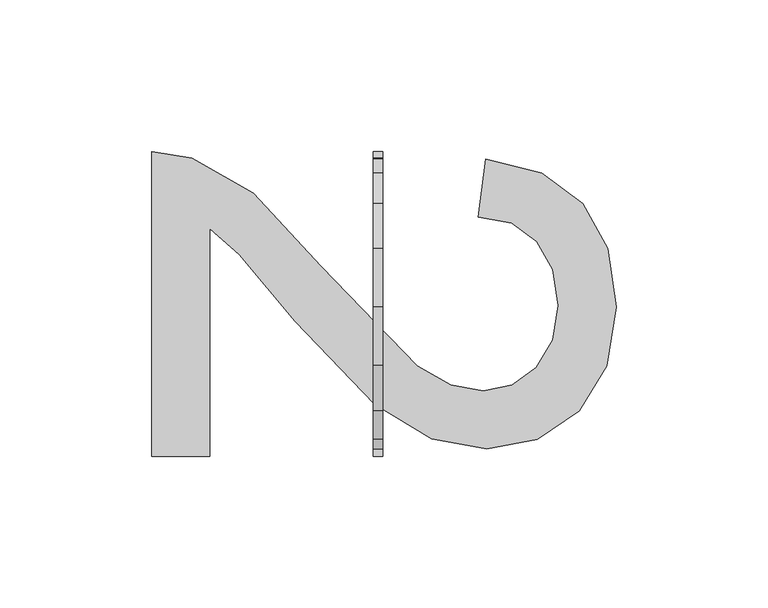
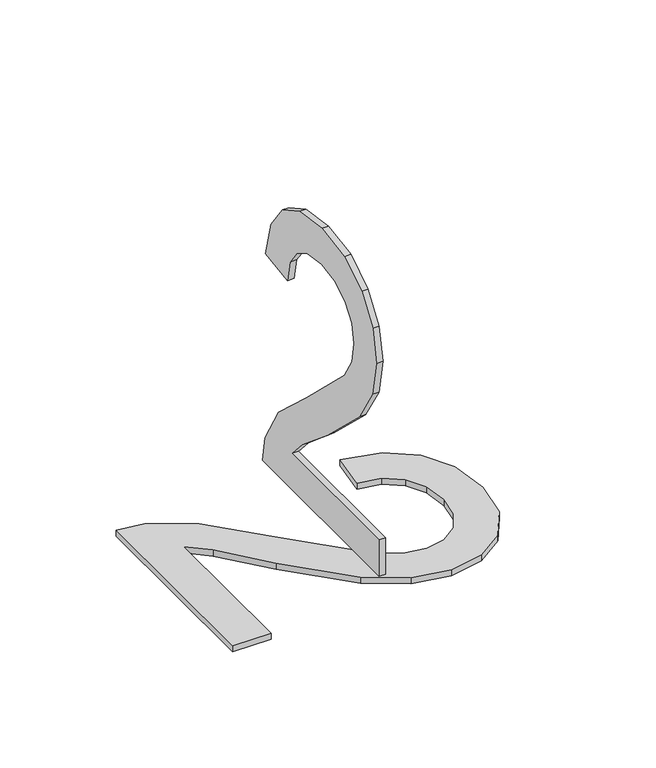
"""IFC4 building model written with IfcOpenShell, lengths in millimetres: proxy geometry, Grid Number2_FedEx : Grid Number2_FedEx."""

from ifc_helpers import new_model, si_unit, frame, origin, origin_with_axes, place, context, project, spatial, polyline, outline, extrude, source, transform, mapped, element, save


def entourage_708554ca(model_context):
    return source(origin(), model_context, "Body", "SweptSolid", [
        extrude(outline(polyline([(-165.1369997, 173.4823009), (-184.2739267, 173.4823009), (-184.2739267, 273.9511681), (-171.0799126, 271.8954435), (-150.7656159, 260.2712553), (-128.5824788, 236.3127197), (-96.7000592, 203.271619), (-85.7112769, 197.0764126), (-75.021509, 195.0113438), (-65.4390292, 196.9596101), (-57.4730964, 202.8044089), (-52.104852, 211.7888597), (-50.3154372, 223.1560823), (-52.0628031, 235.0933012), (-57.3049008, 244.3674224), (-65.6305853, 250.3523842), (-76.6287119, 252.4221251), (-74.236596, 271.5590522), (-55.7257305, 266.9196555), (-42.2046692, 256.888654), (-33.9350499, 241.9893228), (-31.1785101, 222.7449374), (-34.2434085, 203.3603889), (-43.438104, 188.4890904), (-57.1740819, 179.0280852), (-73.8628279, 175.8744168), (-92.0092695, 179.2757065), (-110.7724285, 190.5821918), (-136.9922612, 217.9980824), (-155.4003405, 240.0130239), (-165.1369997, 248.6470672), (-165.1369997, 173.4823009)])), origin_with_axes(), (0.0, 0.0, 1.0), 3.175),
        extrude(outline(polyline([(173.4823009, 33.3752024), (248.6470672, 33.3752024), (240.0130239, 43.1118616), (217.9980824, 61.5199409), (190.5821918, 87.7397736), (179.2757065, 106.5029325), (175.8744168, 124.6493741), (179.0280852, 141.3381201), (188.4890904, 155.0740981), (203.3603889, 164.2687935), (222.7449374, 167.333692), (241.9893228, 164.5771522), (256.888654, 156.3075328), (266.9196555, 142.7864715), (271.5590522, 124.275606), (252.4221251, 121.8834901), (250.3523842, 132.8816167), (244.3674224, 141.2073013), (235.0933012, 146.449399), (223.1560823, 148.1967649), (211.7888597, 146.4073501), (202.8044089, 141.0391056), (196.9596101, 133.0731729), (195.0113438, 123.490693), (197.0764126, 112.8009251), (203.271619, 101.8121428), (236.3127197, 69.9297233), (260.2712553, 47.7465861), (271.8954435, 27.4322895), (273.9511681, 14.2382753), (173.4823009, 14.2382753), (173.4823009, 33.3752024)])), frame((-111.2489267, 0.0, 0.0), z_axis=(1.0, 0.0, 0.0), x_axis=(0.0, 1.0, 0.0)), (0.0, 0.0, 1.0), 3.175),
    ])


if __name__ == "__main__":
    model = new_model("IFC4")
    model_context = context("Model", 3, world=origin())
    ifc_project = project(units=[si_unit("LENGTHUNIT", "METRE", prefix="MILLI")], contexts=[model_context])
    site = spatial("IfcSite", under=ifc_project)
    building = spatial("IfcBuilding", under=site)
    placement = place(None, origin())
    entourage_shape = entourage_708554ca(model_context)
    element("IfcBuildingElementProxy", 1, Name="Grid Number2_FedEx : Grid Number2_FedEx", ObjectType="Grid Number2_FedEx : Grid Number2_FedEx", at=placement, inside=building, context=model_context, shape_type="MappedRepresentation", body=[
        mapped(entourage_shape, transform((0.0, 0.0, 0.0), x_axis=(1.0, 0.0, 0.0), y_axis=(0.0, 1.0, 0.0), z_axis=(0.0, 0.0, 1.0))),
    ])
    save(model, "model.ifc")

# Revit data of these elements
# Type "Grid Number2_FedEx : Grid Number2_FedEx"
#   Grid [instance default] = "S"
#   Label Width [instance default] = 1' - 0"
#   Half Box Width2 [instance default] = 0' - 6.13846"
#   Half Box Width [instance default] = 0' - 6"
#   Robust [instance default] = yes
#   Height = 0
#   Assembly Code = ""
# Element 1 (IfcBuildingElementProxy, "Grid Number2_FedEx : Grid Number2_FedEx")
#   Grid = "2"
#   Robust = no
#   Materials on its faces: "Letter"
# Materials
#   "Letter": class "Unassigned", colour RGB 178 187 30, transparency 0, Comments = "Rendering appearance not upgraded "
